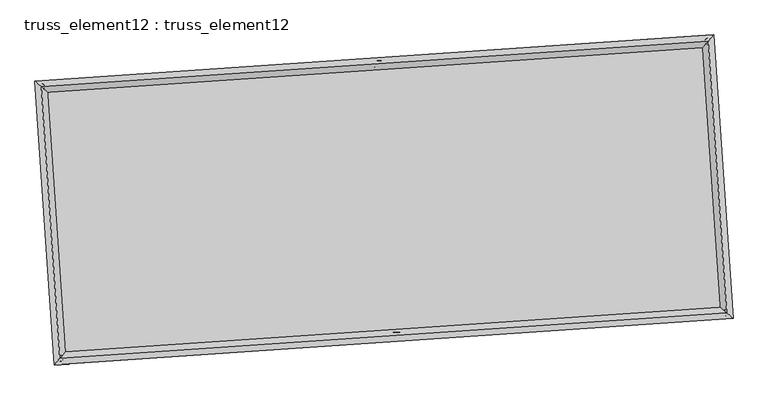
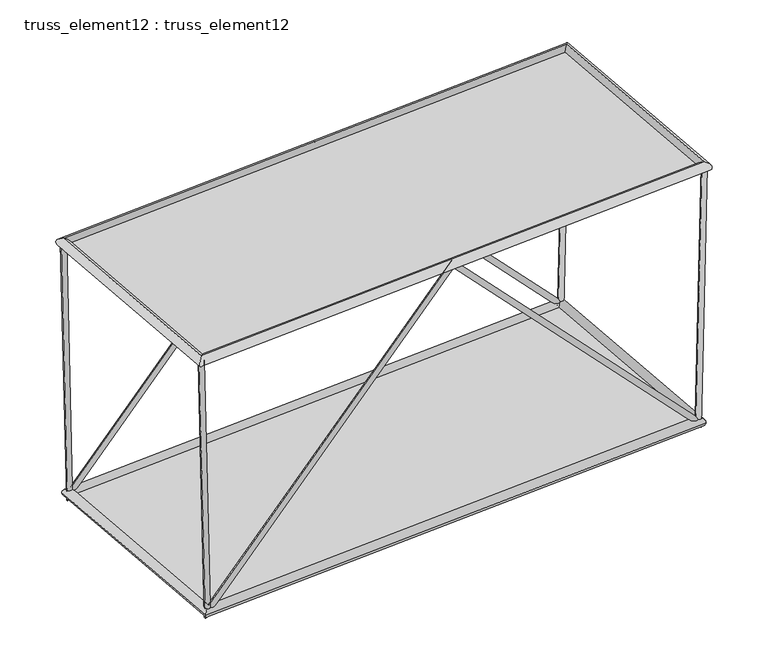
"""IFC4 building model written with IfcOpenShell, lengths in millimetres: plate geometry, truss_element12 : truss_element12."""

from ifc_helpers import new_model, si_unit, frame, origin, origin_with_axes, place, context, project, spatial, polyline, circle_curve, ellipse_curve, outline, extrude, source, transform, mapped, element, save
from ifc_brep_helpers import plane_surface, cylinder_surface, advanced_brep


def truss_element12_truss_element12_a9ba9ad0(model_context):
    return source(origin(), model_context, "Body", "SolidModel", [
        advanced_brep(
        [(-3781.0066057, 2268.3099305, 4999.8074441), (-3880.0830312, 2254.9505451, 4997.4860818), (-3667.7432726, 2276.0329266, 121.2492765), (-3761.2436102, 2263.0537535, -121.2492765), (1063.9114307, 2598.6664741, 5070.7560558), (1064.3567641, 2592.0930992, 4926.5285654), (5795.1912206, 2921.2744577, 121.2466741), (5889.5697565, 2921.1060308, -121.2466741), (5908.826689, 2929.0228283, 4999.8023514), (6008.7993375, 2929.2358427, 4997.4733651)],
        [
            (0, 1, circle_curve(frame((-3830.5448184, 2261.6302378, 4998.6467629), z_axis=(-0.023210275405575107, -0.0015826204493892785, 0.9997293525890447), x_axis=(-0.1335944347975753, 0.9910349023519434, -0.0015327463556159752)), 50.0)),
            (1, 0, circle_curve(frame((-3830.5448184, 2261.6302378, 4998.6467629), z_axis=(-0.023210275405575107, -0.0015826204493892785, 0.9997293525890447), x_axis=(-0.1335944347975753, 0.9910349023519434, -0.0015327463556159752)), 50.0)),
            (0, 2),
            (2, 3, ellipse_curve(frame((-3714.4934414, 2269.54334, 0.0), z_axis=(-0.9300246539008389, -0.06341484579481178, 0.3619843925771457), x_axis=(0.36114581811246804, 0.024625160493310073, 0.9321841553741164)), 130.3533132, 50.0)),
            (3, 1),
            (3, 2, ellipse_curve(frame((-3714.4934414, 2269.54334, 0.0), z_axis=(-0.9300246539008389, -0.06341484579481178, 0.3619843925771457), x_axis=(0.36114581811246804, 0.024625160493310073, 0.9321841553741164)), 130.3533132, 50.0)),
            (2, 4),
            (4, 5, ellipse_curve(frame((1064.1340974, 2595.3797867, 4998.6423106), z_axis=(-0.9976833958768766, -0.06802823821520107, 1.99228329783538e-05), x_axis=(-1.9876679665461313e-05, -1.3553152281554114e-06, -0.9999999998015403)), 72.2707708, 50.0)),
            (5, 3),
            (5, 4, ellipse_curve(frame((1064.1340974, 2595.3797867, 4998.6423106), z_axis=(-0.9976833958768766, -0.06802823821520107, 1.99228329783538e-05), x_axis=(-1.9876679665461313e-05, -1.3553152281554114e-06, -0.9999999998015403)), 72.2707708, 50.0)),
            (4, 6),
            (6, 7, ellipse_curve(frame((5842.3804885, 2921.1902443, 0.0), z_axis=(-0.930045648078386, -0.06341627730797217, -0.36193019805323456), x_axis=(-0.3610917491358036, -0.02462147373532669, 0.9322051982997877)), 130.347573, 50.0)),
            (7, 5),
            (7, 6, ellipse_curve(frame((5842.3804885, 2921.1902443, 0.0), z_axis=(-0.930045648078386, -0.06341627730797217, -0.36193019805323456), x_axis=(-0.3610917491358036, -0.02462147373532669, 0.9322051982997877)), 130.347573, 50.0)),
            (8, 9, circle_curve(frame((5958.8130133, 2929.1293355, 4998.6378583), z_axis=(0.023286504957413055, 0.001587818252753427, 0.9997275716514297), x_axis=(-0.002166543517392095, 0.9999964706541518, -0.0015377803573986969)), 50.0)),
            (9, 8, circle_curve(frame((5958.8130133, 2929.1293355, 4998.6378583), z_axis=(0.023286504957413055, 0.001587818252753427, 0.9997275716514297), x_axis=(-0.002166543517392095, 0.9999964706541518, -0.0015377803573986969)), 50.0)),
            (6, 8),
            (9, 7),
        ],
        [
            plane_surface(frame((-3830.5448184, 2311.6301752, 4998.7259153), z_axis=(-0.023210275405573556, -0.0015826204493892511, 0.9997293525890448), x_axis=(0.9997306052710387, -3.674295485112113e-05, 0.023210246322644693))),
            cylinder_surface(frame((-3830.5448184, 2261.6302378, 4998.6467629), z_axis=(-0.02321027540557511, -0.001582620449389279, 0.9997293525890449), x_axis=(-0.1335944347975753, 0.9910349023519434, -0.0015327463556159752)), 50.0),
            cylinder_surface(frame((-3714.4934414, 2269.54334, 0.0), z_axis=(-0.6902542548350474, -0.04706581373513176, -0.7220345371653379), x_axis=(-0.02041980494214943, 0.9987518501447402, -0.04558259973480142)), 50.0),
            cylinder_surface(frame((1064.1340974, 2595.3797867, 4998.6423106), z_axis=(-0.6902255509886974, -0.04706385652896254, 0.7220621040956036), x_axis=(-0.11534286833238303, 0.9922794072885053, -0.04558070420727685)), 50.0),
            plane_surface(frame((5958.8130133, 2879.1293986, 4998.7172707), z_axis=(0.023286504957412656, 0.0015878182527521501, 0.99972757165143), x_axis=(0.9997288325775489, -3.698476667857163e-05, -0.023286475586886003))),
            cylinder_surface(frame((5842.3804885, 2921.1902443, 0.0), z_axis=(-0.023286504957413058, -0.0015878182527534275, -0.9997275716514299), x_axis=(-0.002166543517392095, 0.9999964706541518, -0.0015377803573986969)), 50.0),
        ],
        [
            (0, [[1, 2]]),
            (1, [[-1, 3, 4, 5]]),
            (1, [[-2, -5, 6, -3]]),
            (2, [[-4, 7, 8, 9]]),
            (2, [[-6, -9, 10, -7]]),
            (3, [[-8, 11, 12, 13]]),
            (3, [[-10, -13, 14, -11]]),
            (4, [[15, 16]]),
            (5, [[-12, 17, -16, 18]]),
            (5, [[-14, -18, -15, -17]]),
        ],
    ),
        advanced_brep(
        [(-3508.8936528, -1722.4236538, 4999.8074441), (-3607.9700783, -1735.7830392, 4997.4860818), (-3395.6303197, -1714.7006577, 121.2492765), (-3489.1306573, -1727.6798308, -121.2492765), (1336.0243837, -1392.0671102, 5070.7560558), (1336.469717, -1398.6404851, 4926.5285654), (6067.3041735, -1069.4591266, 121.2466741), (6161.6827094, -1069.6275535, -121.2466741), (6180.939642, -1061.710756, 4999.8023514), (6280.9122905, -1061.4977416, 4997.4733651)],
        [
            (0, 1, circle_curve(frame((-3558.4318655, -1729.1033465, 4998.6467629), z_axis=(-0.023210275405574413, -0.001582620449389233, 0.9997293525890448), x_axis=(-0.13359443479757582, 0.9910349023519432, -0.0015327463556159403)), 50.0)),
            (1, 0, circle_curve(frame((-3558.4318655, -1729.1033465, 4998.6467629), z_axis=(-0.023210275405574413, -0.001582620449389233, 0.9997293525890448), x_axis=(-0.13359443479757582, 0.9910349023519432, -0.0015327463556159403)), 50.0)),
            (0, 2),
            (2, 3, ellipse_curve(frame((-3442.3804885, -1721.1902443, 0.0), z_axis=(-0.9300246539008385, -0.06341484579481202, 0.36198439257714643), x_axis=(0.3611458181124687, 0.024625160493310223, 0.9321841553741161)), 130.3533132, 50.0)),
            (3, 1),
            (3, 2, ellipse_curve(frame((-3442.3804885, -1721.1902443, 0.0), z_axis=(-0.9300246539008385, -0.06341484579481202, 0.36198439257714643), x_axis=(0.3611458181124687, 0.024625160493310223, 0.9321841553741161)), 130.3533132, 50.0)),
            (2, 4),
            (4, 5, ellipse_curve(frame((1336.2470503, -1395.3537976, 4998.6423106), z_axis=(-0.9976833958768766, -0.06802823821520144, 1.9922832978915455e-05), x_axis=(-1.9876679665922593e-05, -1.3553152280977514e-06, -0.9999999998015403)), 72.2707708, 50.0)),
            (5, 3),
            (5, 4, ellipse_curve(frame((1336.2470503, -1395.3537976, 4998.6423106), z_axis=(-0.9976833958768766, -0.06802823821520144, 1.9922832978915455e-05), x_axis=(-1.9876679665922593e-05, -1.3553152280977514e-06, -0.9999999998015403)), 72.2707708, 50.0)),
            (4, 6),
            (6, 7, ellipse_curve(frame((6114.4934414, -1069.54334, 0.0), z_axis=(-0.930045648078386, -0.0634162773079726, -0.36193019805323406), x_axis=(-0.3610917491358033, -0.02462147373532683, 0.9322051982997878)), 130.347573, 50.0)),
            (7, 5),
            (7, 6, ellipse_curve(frame((6114.4934414, -1069.54334, 0.0), z_axis=(-0.930045648078386, -0.0634162773079726, -0.36193019805323406), x_axis=(-0.3610917491358033, -0.02462147373532683, 0.9322051982997878)), 130.347573, 50.0)),
            (8, 9, circle_curve(frame((6230.9259662, -1061.6042488, 4998.6378583), z_axis=(0.023286504957413627, 0.0015878182527534774, 0.9997275716514298), x_axis=(-0.0021665435173920953, 0.9999964706541518, -0.0015377803573987457)), 50.0)),
            (9, 8, circle_curve(frame((6230.9259662, -1061.6042488, 4998.6378583), z_axis=(0.023286504957413627, 0.0015878182527534774, 0.9997275716514298), x_axis=(-0.0021665435173920953, 0.9999964706541518, -0.0015377803573987457)), 50.0)),
            (6, 8),
            (9, 7),
        ],
        [
            plane_surface(frame((-3558.4318655, -1679.1034091, 4998.7259153), z_axis=(-0.023210275405573556, -0.0015826204493892427, 0.9997293525890448), x_axis=(0.9997306052710387, -3.674295485112113e-05, 0.023210246322644693))),
            cylinder_surface(frame((-3558.4318655, -1729.1033465, 4998.6467629), z_axis=(-0.023210275405574413, -0.001582620449389233, 0.9997293525890448), x_axis=(-0.13359443479757582, 0.9910349023519432, -0.0015327463556159403)), 50.0),
            cylinder_surface(frame((-3442.3804885, -1721.1902443, 0.0), z_axis=(-0.6902542548350478, -0.04706581373513197, -0.7220345371653374), x_axis=(-0.020419804942149452, 0.9987518501447401, -0.0455825997348017)), 50.0),
            cylinder_surface(frame((1336.2470503, -1395.3537976, 4998.6423106), z_axis=(-0.6902255509886973, -0.04706385652896285, 0.7220621040956039), x_axis=(-0.11534286833238368, 0.9922794072885052, -0.04558070420727702)), 50.0),
            plane_surface(frame((6230.9259662, -1111.6041857, 4998.7172707), z_axis=(0.023286504957412656, 0.001587818252752135, 0.99972757165143), x_axis=(0.9997288325775489, -3.698476667812754e-05, -0.023286475586886003))),
            cylinder_surface(frame((6114.4934414, -1069.54334, 0.0), z_axis=(-0.023286504957413627, -0.0015878182527534774, -0.9997275716514298), x_axis=(-0.0021665435173920953, 0.9999964706541518, -0.0015377803573987457)), 50.0),
        ],
        [
            (0, [[1, 2]]),
            (1, [[-1, 3, 4, 5]]),
            (1, [[-2, -5, 6, -3]]),
            (2, [[-4, 7, 8, 9]]),
            (2, [[-6, -9, 10, -7]]),
            (3, [[-8, 11, 12, 13]]),
            (3, [[-10, -13, 14, -11]]),
            (4, [[15, 16]]),
            (5, [[-12, 17, -16, 18]]),
            (5, [[-14, -18, -15, -17]]),
        ],
    ),
        advanced_brep(
        [(-3558.4341768, -1729.1059081, 4908.646763), (-3558.4295543, -1729.1007848, 5088.6467629), (-3830.5421809, 2261.6280136, 5088.6467629), (-3830.547456, 2261.632462, 4908.646763), (5958.810865, 2929.126785, 5088.6378582), (5958.8151616, 2929.1318861, 4908.6378583), (6230.9234916, -1061.6020135, 5088.6378582), (6230.9284408, -1061.6064841, 4908.6378583)],
        [
            (0, 1, ellipse_curve(frame((-3558.4318655, -1729.1033465, 4998.6467629), z_axis=(-0.7535719234051691, 0.6573654662780984, 6.417150933687899e-07), x_axis=(-0.657365466277788, -0.7535719234054401, 6.417150933687674e-07)), 127.2792206, 90.0)),
            (1, 2),
            (2, 3, ellipse_curve(frame((-3830.5448184, 2261.6302378, 4998.6467629), z_axis=(-0.6573654662777882, -0.7535719234054399, 6.417150933687475e-07), x_axis=(0.753571923405169, -0.6573654662780987, -6.417150933687697e-07)), 127.2792206, 90.0)),
            (3, 0),
            (1, 0, ellipse_curve(frame((-3558.4318655, -1729.1033465, 4998.6467629), z_axis=(-0.7535719234051691, 0.6573654662780984, 6.417150933687899e-07), x_axis=(-0.657365466277788, -0.7535719234054401, 6.417150933687674e-07)), 127.2792206, 90.0)),
            (3, 2, ellipse_curve(frame((-3830.5448184, 2261.6302378, 4998.6467629), z_axis=(-0.6573654662777882, -0.7535719234054399, 6.417150933687475e-07), x_axis=(0.753571923405169, -0.6573654662780987, -6.417150933687697e-07)), 127.2792206, 90.0)),
            (2, 4),
            (4, 5, ellipse_curve(frame((5958.8130133, 2929.1293355, 4998.6378583), z_axis=(-0.7535719234051688, 0.6573654662780991, 6.417150933687491e-07), x_axis=(-0.6573654662777887, -0.7535719234054395, 6.417150933687683e-07)), 127.2792206, 90.0)),
            (5, 3),
            (5, 4, ellipse_curve(frame((5958.8130133, 2929.1293355, 4998.6378583), z_axis=(-0.7535719234051688, 0.6573654662780991, 6.417150933687491e-07), x_axis=(-0.6573654662777887, -0.7535719234054395, 6.417150933687683e-07)), 127.2792206, 90.0)),
            (4, 6),
            (6, 7, ellipse_curve(frame((6230.9259662, -1061.6042488, 4998.6378583), z_axis=(0.6573654662777887, 0.7535719234054394, -6.417150933687883e-07), x_axis=(-0.7535719234051687, 0.6573654662780992, 6.41715093368769e-07)), 127.2792206, 90.0)),
            (7, 5),
            (7, 6, ellipse_curve(frame((6230.9259662, -1061.6042488, 4998.6378583), z_axis=(0.6573654662777887, 0.7535719234054394, -6.417150933687883e-07), x_axis=(-0.7535719234051687, 0.6573654662780992, 6.41715093368769e-07)), 127.2792206, 90.0)),
            (6, 1),
            (0, 7),
        ],
        [
            cylinder_surface(frame((-3558.4318655, -1729.1033465, 4998.6467629), z_axis=(0.0680282382287046, -0.9976833960748763, 0.0), x_axis=(-0.9976833956960517, -0.068028238202874, 2.7557367220821674e-05)), 90.0),
            cylinder_surface(frame((-3830.5448184, 2261.6302378, 4998.6467629), z_axis=(-0.9976833960744657, -0.06802823822867518, 9.075221882216156e-07), x_axis=(-0.06802823818041658, 0.9976833957222373, 2.6649845032922314e-05)), 90.0),
            cylinder_surface(frame((5958.8130133, 2929.1293355, 4998.6378583), z_axis=(-0.06802823822870338, 0.9976833960748765, 0.0), x_axis=(0.9976833957443104, 0.06802823820616334, 2.5742322845022958e-05)), 90.0),
            cylinder_surface(frame((6230.9259662, -1061.6042488, 4998.6378583), z_axis=(0.9976833960744657, 0.06802823822867522, -9.07522188221644e-07), x_axis=(0.06802823822867522, -0.9976833957189467, 2.6649845032922317e-05)), 90.0),
        ],
        [
            (0, [[1, 2, 3, 4]]),
            (0, [[5, -4, 6, -2]]),
            (1, [[-3, 7, 8, 9]]),
            (1, [[-6, -9, 10, -7]]),
            (2, [[-8, 11, 12, 13]]),
            (2, [[-10, -13, 14, -11]]),
            (3, [[-12, 15, -1, 16]]),
            (3, [[-14, -16, -5, -15]]),
        ],
    ),
        advanced_brep(
        [(-3358.7115243, -1625.2761972, 0.0), (-3526.0494527, -1817.1042913, 0.0), (-3810.4074885, 2353.2123043, 0.0), (-3618.5793943, 2185.8743758, 0.0), (5926.0494527, 3017.1042913, 0.0), (5758.7115243, 2825.2761972, 0.0), (6210.4074885, -1153.2123043, 0.0), (6018.5793943, -985.8743758, 0.0)],
        [
            (0, 1, ellipse_curve(frame((-3442.3804885, -1721.1902443, 0.0), z_axis=(-0.7535719234054589, 0.6573654662780797, 0.0), x_axis=(-0.6573654662780796, -0.753571923405459, 0.0)), 127.2792206, 90.0)),
            (1, 2),
            (2, 3, ellipse_curve(frame((-3714.4934414, 2269.54334, 0.0), z_axis=(-0.6573654662780798, -0.7535719234054586, 0.0), x_axis=(0.7535719234054585, -0.6573654662780801, 0.0)), 127.2792206, 90.0)),
            (3, 0),
            (1, 0, ellipse_curve(frame((-3442.3804885, -1721.1902443, 0.0), z_axis=(-0.7535719234054589, 0.6573654662780797, 0.0), x_axis=(-0.6573654662780796, -0.753571923405459, 0.0)), 127.2792206, 90.0)),
            (3, 2, ellipse_curve(frame((-3714.4934414, 2269.54334, 0.0), z_axis=(-0.6573654662780798, -0.7535719234054586, 0.0), x_axis=(0.7535719234054585, -0.6573654662780801, 0.0)), 127.2792206, 90.0)),
            (2, 4),
            (4, 5, ellipse_curve(frame((5842.3804885, 2921.1902443, 0.0), z_axis=(-0.7535719234054585, 0.6573654662780802, 0.0), x_axis=(-0.6573654662780801, -0.7535719234054584, 0.0)), 127.2792206, 90.0)),
            (5, 3),
            (5, 4, ellipse_curve(frame((5842.3804885, 2921.1902443, 0.0), z_axis=(-0.7535719234054585, 0.6573654662780802, 0.0), x_axis=(-0.6573654662780801, -0.7535719234054584, 0.0)), 127.2792206, 90.0)),
            (4, 6),
            (6, 7, ellipse_curve(frame((6114.4934414, -1069.54334, 0.0), z_axis=(0.65736546627808, 0.7535719234054586, 0.0), x_axis=(-0.7535719234054588, 0.6573654662780799, 0.0)), 127.2792206, 90.0)),
            (7, 5),
            (7, 6, ellipse_curve(frame((6114.4934414, -1069.54334, 0.0), z_axis=(0.65736546627808, 0.7535719234054586, 0.0), x_axis=(-0.7535719234054588, 0.6573654662780799, 0.0)), 127.2792206, 90.0)),
            (6, 1),
            (0, 7),
        ],
        [
            cylinder_surface(frame((-3442.3804885, -1721.1902443, 0.0), z_axis=(0.068028238228703, -0.9976833960748764, 0.0), x_axis=(-0.9976833960748764, -0.068028238228703, 0.0)), 90.0),
            cylinder_surface(frame((-3714.4934414, 2269.54334, 0.0), z_axis=(-0.9976833960748765, -0.06802823822870191, 0.0), x_axis=(-0.06802823822870191, 0.9976833960748765, 0.0)), 90.0),
            cylinder_surface(frame((5842.3804885, 2921.1902443, 0.0), z_axis=(-0.06802823822870221, 0.9976833960748765, 0.0), x_axis=(0.9976833960748765, 0.06802823822870221, 0.0)), 90.0),
            cylinder_surface(frame((6114.4934414, -1069.54334, 0.0), z_axis=(0.9976833960748765, 0.0680282382287023, 0.0), x_axis=(0.0680282382287023, -0.9976833960748765, 0.0)), 90.0),
        ],
        [
            (0, [[1, 2, 3, 4]]),
            (0, [[5, -4, 6, -2]]),
            (1, [[-3, 7, 8, 9]]),
            (1, [[-6, -9, 10, -7]]),
            (2, [[-8, 11, 12, 13]]),
            (2, [[-10, -13, 14, -11]]),
            (3, [[-12, 15, -1, 16]]),
            (3, [[-14, -16, -5, -15]]),
        ],
    ),
        extrude(outline(polyline([(-3442.3804885, -1721.1902443), (-3714.4934414, 2269.54334), (5842.3804885, 2921.1902443), (6114.4934414, -1069.54334), (-3442.3804885, -1721.1902443)])), origin_with_axes(), (0.0, 0.0, 1.0), 20.0),
        extrude(outline(polyline([(-2000.0, 4906.0442773), (2000.0, 4906.0442773), (2000.0, -4906.0442773), (-2000.0, -4906.0442773), (-2000.0, 4906.0442773)])), frame((1200.1905739, 600.0129945, 4998.6423106), z_axis=(9.054198187582591e-07, 6.173713561817491e-08, 0.9999999999995882), x_axis=(-0.068028238228703, 0.9976833960748764, 0.0)), (0.0, 0.0, 1.0), 20.0),
    ])


if __name__ == "__main__":
    model = new_model("IFC4")
    model_context = context("Model", 3, world=origin())
    ifc_project = project(units=[si_unit("LENGTHUNIT", "METRE", prefix="MILLI")], contexts=[model_context])
    site = spatial("IfcSite", under=ifc_project)
    building = spatial("IfcBuilding", under=site)
    placement = place(None, origin())
    truss_element12_truss_element12_shape = truss_element12_truss_element12_a9ba9ad0(model_context)
    element("IfcPlate", 1, ObjectType="truss_element12 : truss_element12", at=placement, inside=building, context=model_context, shape_type="MappedRepresentation", body=[
        mapped(truss_element12_truss_element12_shape, transform((0.0, 0.0, 0.0), x_axis=(1.0, 0.0, 0.0), y_axis=(0.0, 1.0, 0.0), z_axis=(0.0, 0.0, 1.0))),
    ])
    save(model, "model.ifc")

# Revit data of these elements
# Type "truss_element12 : truss_element12"
#   steellbar1 = 90 mm
#   steelbar2 = 50 mm
#   offset1 = 5000 mm
#   M = Default Roof
# Element 1 (IfcPlate, "truss_element12 : truss_element12")
#   Materials on its faces: "Default Roof"
# Materials
#   "Default Roof": class "Miscellaneous", colour RGB 0 127 0, transparency 0, Comments = "Rendering appearance not upgraded Rendering appearance not upgraded ", Cost = 0
